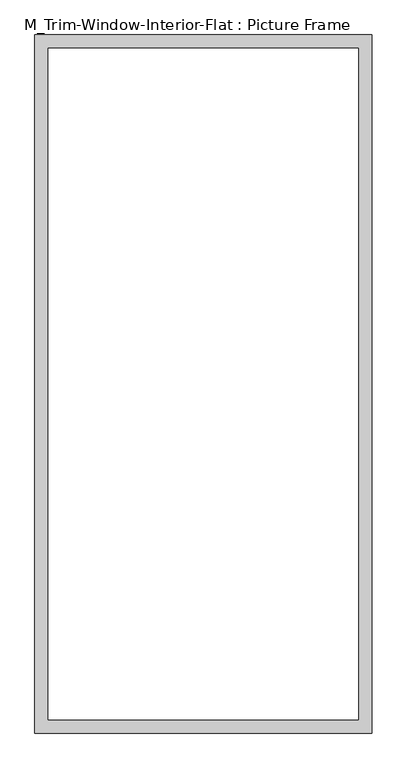
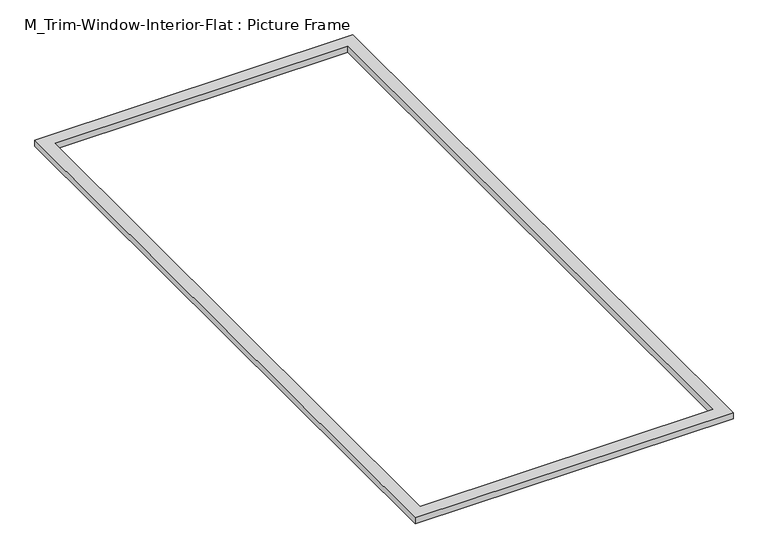
"""IFC4 building model written with IfcOpenShell, lengths in millimetres: proxy geometry, M_Trim-Window-Interior-Flat : Picture Frame."""

from ifc_helpers import new_model, si_unit, origin, origin_with_axes, place, context, project, spatial, polyline, outline, extrude, source, transform, mapped, element, save


def m_trim_window_interior_flat_picture_frame_0cdd5c6c(model_context):
    return source(origin(), model_context, "Body", "SweptSolid", [
        extrude(outline(polyline([(747.3, 47.3), (747.3, -3047.3), (-747.3, -3047.3), (-747.3, 47.3), (747.3, 47.3)]), holes=[polyline([(687.3, -12.7), (-687.3, -12.7), (-687.3, -2987.3), (687.3, -2987.3), (687.3, -12.7)])]), origin_with_axes(), (0.0, 0.0, 1.0), 30.0),
    ])


if __name__ == "__main__":
    model = new_model("IFC4")
    model_context = context("Model", 3, world=origin())
    ifc_project = project(units=[si_unit("LENGTHUNIT", "METRE", prefix="MILLI")], contexts=[model_context])
    site = spatial("IfcSite", under=ifc_project)
    building = spatial("IfcBuilding", under=site)
    placement = place(None, origin())
    m_trim_window_interior_flat_picture_frame_shape = m_trim_window_interior_flat_picture_frame_0cdd5c6c(model_context)
    element("IfcBuildingElementProxy", 1, Name="M_Trim-Window-Interior-Flat : Picture Frame", ObjectType="M_Trim-Window-Interior-Flat : Picture Frame", at=placement, inside=building, context=model_context, shape_type="MappedRepresentation", body=[
        mapped(m_trim_window_interior_flat_picture_frame_shape, transform((0.0, 0.0, 0.0), x_axis=(1.0, 0.0, 0.0), y_axis=(0.0, 1.0, 0.0), z_axis=(0.0, 0.0, 1.0))),
    ])
    save(model, "model.ifc")

# Revit data of these elements
# Type "M_Trim-Window-Interior-Flat : Picture Frame"
#   Trim Thickness_Picture Frame = 30 mm
#   Trim Width = 60 mm
#   Trim Thickness_with Sill = 20 mm
#   Sill Thickness = 30 mm
#   Opening Width [instance default] = 600 mm
#   Opening Height [instance default] = 900 mm
#   Default Elevation = 1200 mm
#   Sill = no
#   Picture Frame = yes
#   Trim Material [instance default] = none
# Element 1 (IfcBuildingElementProxy, "M_Trim-Window-Interior-Flat : Picture Frame")
#   Opening Width = 1400 mm
#   Opening Height = 3000 mm
#   Trim Material = Wood - Stained
#   Materials on its faces: "Wood - Stained"
# Materials
#   "Wood - Stained": class "Wood", colour RGB 173 132 96, transparency 0, Cost = 0
